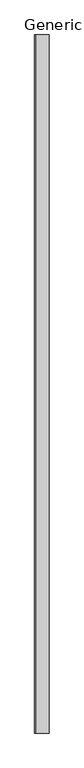
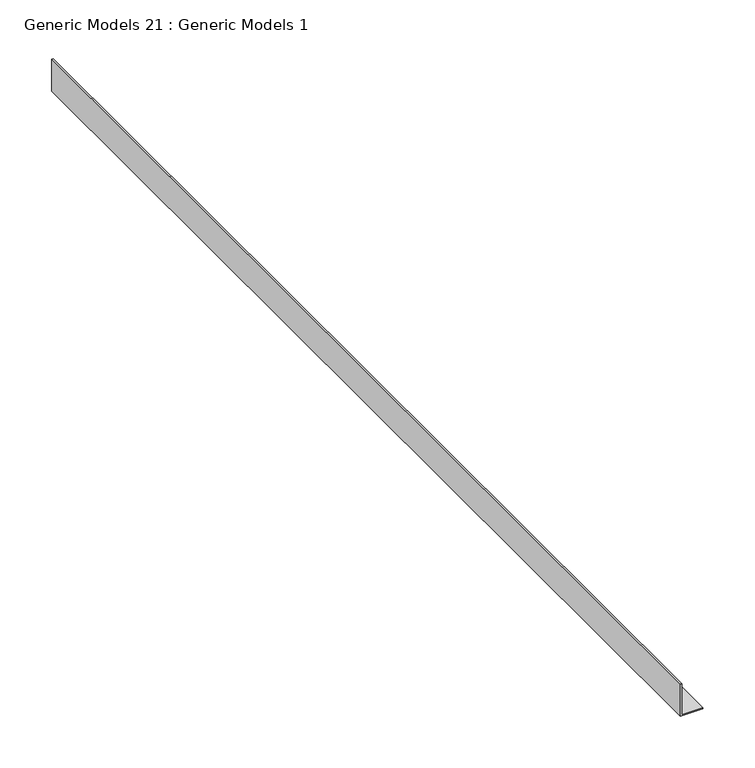
"""IFC4 building model written with IfcOpenShell, lengths in millimetres: proxy geometry, Generic Models 21 : Generic Models 1."""

from ifc_helpers import new_model, si_unit, frame, origin, place, context, project, spatial, polyline, outline, extrude, source, transform, mapped, element, save


def generic_models_21_generic_models_1_e8c90d4c(model_context):
    return source(origin(), model_context, "Body", "SweptSolid", [
        extrude(outline(polyline([(2277.1204978, 49799.875), (2239.0204978, 49799.875), (2239.0204978, 49825.275), (2240.6079978, 49825.275), (2240.6079978, 49801.4625), (2277.1204978, 49801.4625), (2277.1204978, 49799.875)])), frame((0.0, 0.0, 0.0), z_axis=(0.0, 1.0, 0.0), x_axis=(0.0, 0.0, 1.0)), (0.0, 0.0, 1.0), 1219.2),
    ])


if __name__ == "__main__":
    model = new_model("IFC4")
    model_context = context("Model", 3, world=origin())
    ifc_project = project(units=[si_unit("LENGTHUNIT", "METRE", prefix="MILLI")], contexts=[model_context])
    site = spatial("IfcSite", under=ifc_project)
    building = spatial("IfcBuilding", under=site)
    placement = place(None, origin())
    generic_models_21_generic_models_1_shape = generic_models_21_generic_models_1_e8c90d4c(model_context)
    element("IfcBuildingElementProxy", 1, Name="Generic Models 21 : Generic Models 1", ObjectType="Generic Models 21 : Generic Models 1", at=placement, inside=building, context=model_context, shape_type="MappedRepresentation", body=[
        mapped(generic_models_21_generic_models_1_shape, transform((0.0, 0.0, 0.0), x_axis=(1.0, 0.0, 0.0), y_axis=(0.0, 1.0, 0.0), z_axis=(0.0, 0.0, 1.0))),
    ])
    save(model, "model.ifc")

# Revit data of these elements
# Element 1 (IfcBuildingElementProxy, "Generic Models 21 : Generic Models 1")
#   Materials on its faces: "CEILING TRACK AS SCHEDULED"
# Materials
#   "CEILING TRACK AS SCHEDULED": class "Unassigned", colour RGB 210 209 208, transparency 0, Keynote = "M05121300.02", Cost = 0
